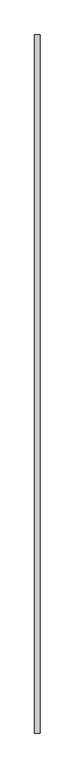
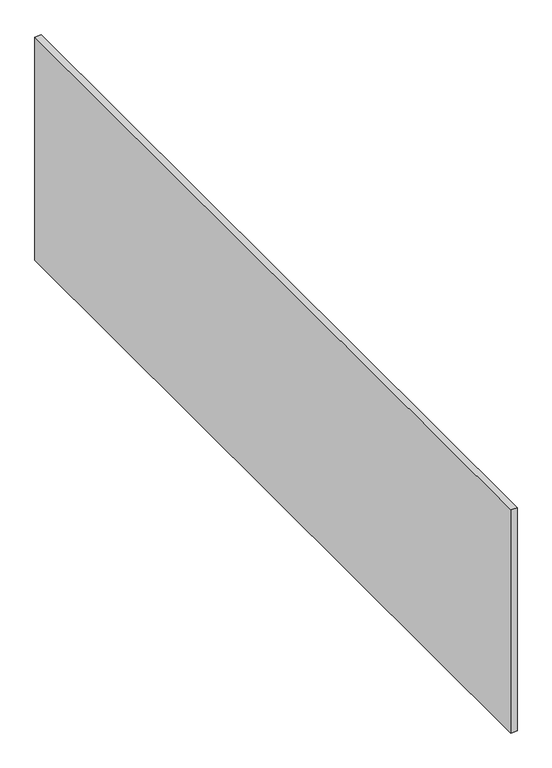
"""IFC4 building model written with IfcOpenShell, lengths in millimetres: proxy geometry, Inner panel:Inner panel:1:Inner panel:1 : Inner panel:Inner panel:300324:300043:Inner panel:1:Inner panel:1 : Inner panel:Inner panel:300324:300043 : Inner panel:Inner panel:1:Inner panel:1 : Inner panel:Inner panel:300324:300043:44 : Inner panel:Inner panel:1:Inner panel:1 : Inner panel:Inner panel:300324:300043:Inner panel:1:Inner panel:1 : Inner panel:Inner panel:300324:300043 : Inner panel:Inner panel:1:Inner panel:1 : Inner panel:Inner panel:300324:300043:300031."""

from ifc_helpers import new_model, si_unit, frame, origin, place, context, project, spatial, polyline, outline, extrude, source, transform, mapped, element, save


def generic_models_d21ff8f6(model_context):
    return source(origin(), model_context, "Body", "SweptSolid", [
        extrude(outline(polyline([(579085.4617239, -576279.7163841), (579104.5117239, -576279.7163841), (579104.5117239, -578718.1163841), (579085.4617239, -578718.1163841), (579085.4617239, -576279.7163841)])), frame((0.0, 0.0, 3745.4990092), z_axis=(0.0, 0.0, 1.0), x_axis=(1.0, 0.0, 0.0)), (0.0, 0.0, 1.0), 699.1241556),
    ])


if __name__ == "__main__":
    model = new_model("IFC4")
    model_context = context("Model", 3, world=origin())
    ifc_project = project(units=[si_unit("LENGTHUNIT", "METRE", prefix="MILLI")], contexts=[model_context])
    site = spatial("IfcSite", under=ifc_project)
    building = spatial("IfcBuilding", under=site)
    placement = place(None, origin())
    generic_models_shape = generic_models_d21ff8f6(model_context)
    element("IfcBuildingElementProxy", 1, Name="Inner panel:Inner panel:1:Inner panel:1 : Inner panel:Inner panel:300324:300043:Inner panel:1:Inner panel:1 : Inner panel:Inner panel:300324:300043 : Inner panel:Inner panel:1:Inner panel:1 : Inner panel:Inner panel:300324:300043:44 : Inner panel:Inner panel:1:Inner panel:1 : Inner panel:Inner panel:300324:300043:Inner panel:1:Inner panel:1 : Inner panel:Inner panel:300324:300043 : Inner panel:Inner panel:1:Inner panel:1 : Inner panel:Inner panel:300324:300043:300031", ObjectType="Inner panel:Inner panel:1:Inner panel:1 : Inner panel:Inner panel:300324:300043:Inner panel:1:Inner panel:1 : Inner panel:Inner panel:300324:300043 : Inner panel:Inner panel:1:Inner panel:1 : Inner panel:Inner panel:300324:300043:44 : Inner panel:Inner panel:1:Inner panel:1 : Inner panel:Inner panel:300324:300043:Inner panel:1:Inner panel:1 : Inner panel:Inner panel:300324:300043 : Inner panel:Inner panel:1:Inner panel:1 : Inner panel:Inner panel:300324:300043:300031", at=placement, inside=building, context=model_context, shape_type="MappedRepresentation", body=[
        mapped(generic_models_shape, transform((0.0, 0.0, 0.0), x_axis=(1.0, 0.0, 0.0), y_axis=(0.0, 1.0, 0.0), z_axis=(0.0, 0.0, 1.0))),
    ])
    save(model, "model.ifc")

# Revit data of these elements
# Type "Inner panel:Inner panel:1:Inner panel:1 : Inner panel:Inner panel:300324:300043:Inner panel:1:Inner panel:1 : Inner panel:Inner panel:300324:300043 : Inner panel:Inner panel:1:Inner panel:1 : Inner panel:Inner panel:300324:300043:44 : Inner panel:Inner panel:1:Inner panel:1 : Inner panel:Inner panel:300324:300043:Inner panel:1:Inner panel:1 : Inner panel:Inner panel:300324:300043 : Inner panel:Inner panel:1:Inner panel:1 : Inner panel:Inner panel:300324:300043:300031"
#   NameOverride = "Inner panel:Inner panel:1:Inner panel:1 : Inner panel:Inner panel:300324:300043:Inner panel:1:Inner panel:1 : Inner panel:Inner panel:300324:300043 : Inner panel:Inner panel:1:Inner panel:1 : Inner panel:Inner panel:300324:300043:300031"
#   ObjectTypeOverride = "Inner panel:1:Inner panel:1 : Inner panel:Inner panel:300324:300043 : Inner panel:Inner panel:1:Inner panel:1 : Inner panel:Inner panel:300324:300043"
#   Reference = "Inner panel"
#   Tag = "300031"
# Element 1 (IfcBuildingElementProxy, "Inner panel:Inner panel:1:Inner panel:1 : Inner panel:Inner panel:300324:300043:Inner panel:1:Inner panel:1 : Inner panel:Inner panel:300324:300043 : Inner panel:Inner panel:1:Inner panel:1 : Inner panel:Inner panel:300324:300043:44 : Inner panel:Inner panel:1:Inner panel:1 : Inner panel:Inner panel:300324:300043:Inner panel:1:Inner panel:1 : Inner panel:Inner panel:300324:300043 : Inner panel:Inner panel:1:Inner panel:1 : Inner panel:Inner panel:300324:300043:300031")
#   Materials on its faces: "¾” (CLASS A) FIRE RETARDANT PLYWOOD ...OR… IF 1/4\" GYP. BD UNDER PLYWOOD, FLAME SPREAD TO BE CLASS C -  (FINISH: GRADE B - PREFINISHED STAINED/SEALED) - 1/4\" GAP BTWN PANELS (FASTENERS T.B.D.)"
# Materials
#   "¾” (CLASS A) FIRE RETARDANT PLYWOOD ...OR… IF 1/4\" GYP. BD UNDER PLYWOOD, FLAME SPREAD TO BE CLASS C -  (FINISH: GRADE B - PREFINISHED STAINED/SEALED) - 1/4\" GAP BTWN PANELS (FASTENERS T.B.D.)": class "Wood", colour RGB 149 120 74, transparency 0, Description = "Plywood, sheathing grade", Cost = 0
